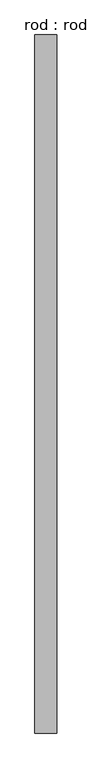
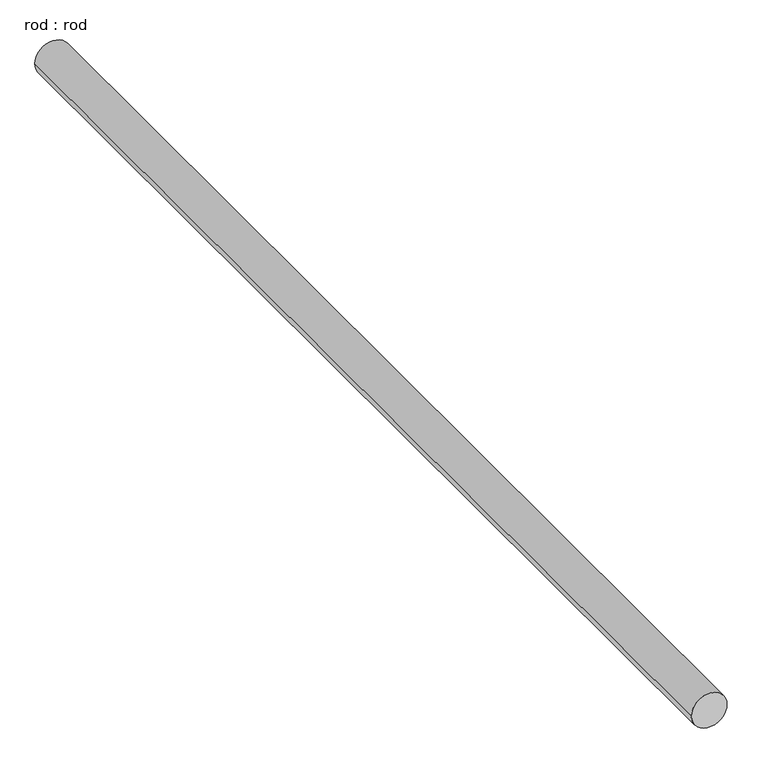
"""IFC4 building model written with IfcOpenShell, lengths in millimetres: proxy geometry, rod : rod."""

from ifc_helpers import new_model, si_unit, point, frame, frame_2d, origin, place, context, project, spatial, circle_curve, trimmed, segment, composite_curve, outline, extrude, source, transform, mapped, element, save


def rod_rod_1a1f919e(model_context):
    return source(origin(), model_context, "Body", "SweptSolid", [
        extrude(outline(composite_curve([segment(trimmed(circle_curve(frame_2d((0.0108462, 0.0)), 200.0), [point((0.0108462, 200.0))], [point((0.0108462, -200.0))], False, "CARTESIAN"), True, "CONTINUOUS"), segment(trimmed(circle_curve(frame_2d((0.0108462, 0.0)), 200.0), [point((0.0108462, -200.0))], [point((0.0108462, 200.0))], False, "CARTESIAN"), True, "CONTINUOUS")], self_intersect=False)), frame((0.0, -2268.3273357, 0.0), z_axis=(0.0, 1.0, 0.0), x_axis=(0.0, 0.0, 1.0)), (0.0, 0.0, 1.0), 12722.1119021),
    ])


if __name__ == "__main__":
    model = new_model("IFC4")
    model_context = context("Model", 3, world=origin())
    ifc_project = project(units=[si_unit("LENGTHUNIT", "METRE", prefix="MILLI")], contexts=[model_context])
    site = spatial("IfcSite", under=ifc_project)
    building = spatial("IfcBuilding", under=site)
    placement = place(None, origin())
    rod_rod_shape = rod_rod_1a1f919e(model_context)
    element("IfcBuildingElementProxy", 1, Name="rod : rod", ObjectType="rod : rod", at=placement, inside=building, context=model_context, shape_type="MappedRepresentation", body=[
        mapped(rod_rod_shape, transform((0.0, 0.0, 0.0), x_axis=(1.0, 0.0, 0.0), y_axis=(0.0, 1.0, 0.0), z_axis=(0.0, 0.0, 1.0))),
    ])
    save(model, "model.ifc")

# Revit data of these elements
# Type "rod : rod"
#   Default Elevation = 0
